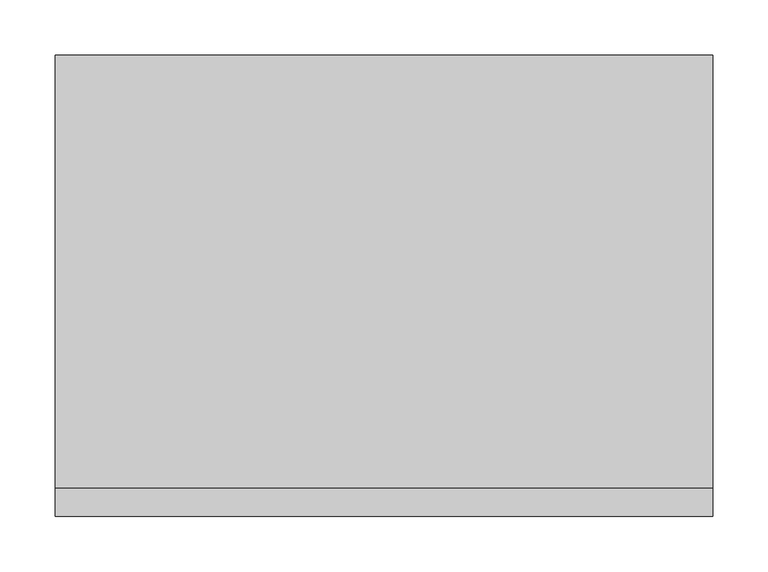
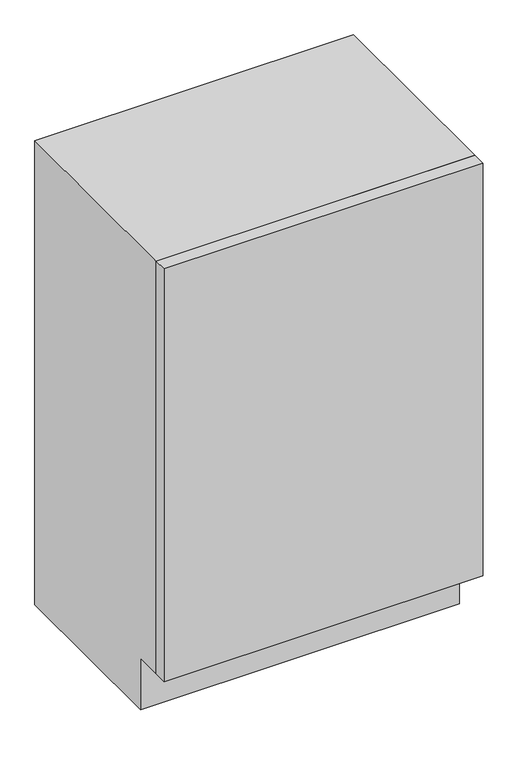
"""IFC4 building model written with IfcOpenShell, lengths in millimetres: furniture geometry, OD_CW_Base Cabinet : OD_CW_Base Cabinet."""

from ifc_helpers import new_model, si_unit, frame, origin, place, context, project, spatial, polyline, outline, extrude, source, transform, mapped, element, save


def furniture_60781b73(model_context):
    return source(origin(), model_context, "Body", "SweptSolid", [
        extrude(outline(polyline([(18.7377049, 217.8726769), (613.1890024, 217.8726769), (613.1890024, 192.4726769), (18.7377049, 192.4726769), (18.7377049, 217.8726769)])), frame((0.0, 0.0, 101.6), z_axis=(0.0, 0.0, 1.0), x_axis=(1.0, 0.0, 0.0)), (0.0, 0.0, 1.0), 812.8),
        extrude(outline(polyline([(217.8726769, 914.4), (609.6, 914.4), (609.6, 0.0), (268.6726769, 0.0), (268.6726769, 101.6), (217.8726769, 101.6), (217.8726769, 914.4)])), frame((18.7377049, 0.0, 0.0), z_axis=(1.0, 0.0, 0.0), x_axis=(0.0, 1.0, 0.0)), (0.0, 0.0, 1.0), 594.4512975),
    ])


if __name__ == "__main__":
    model = new_model("IFC4")
    model_context = context("Model", 3, world=origin())
    ifc_project = project(units=[si_unit("LENGTHUNIT", "METRE", prefix="MILLI")], contexts=[model_context])
    site = spatial("IfcSite", under=ifc_project)
    building = spatial("IfcBuilding", under=site)
    placement = place(None, origin())
    furniture_shape = furniture_60781b73(model_context)
    element("IfcFurniture", 1, ObjectType="OD_CW_Base Cabinet : OD_CW_Base Cabinet", at=placement, inside=building, context=model_context, shape_type="MappedRepresentation", body=[
        mapped(furniture_shape, transform((0.0, 0.0, 0.0), x_axis=(1.0, 0.0, 0.0), y_axis=(0.0, 1.0, 0.0), z_axis=(0.0, 0.0, 1.0))),
    ])
    save(model, "model.ifc")

# Revit data of these elements
# Type "OD_CW_Base Cabinet : OD_CW_Base Cabinet"
#   OD_CW_Width [instance default] = 2' - 10"
#   OD_CW_Length [instance default] = 8' - 0"
#   OD_CW_Height [instance default] = 2' - 3"
#   Depth = 2' - 0"
#   Height = 3' - 0"
#   Width = 4' - 0"
#   OD_CW_Material_Front Panel [instance default] = none
#   OD_CW_Material_Body [instance default] = none
# Element 1 (IfcFurniture, "OD_CW_Base Cabinet : OD_CW_Base Cabinet")
#   OD_CW_Width = 1' - 4.42234"
#   OD_CW_Length = 1' - 11.40359"
#   OD_CW_Height = 3' - 0"
#   Materials on its faces: "CASEWORK"
# Materials
#   "CASEWORK": class "Generic", colour RGB 181 181 181, transparency 0, Cost = 0
